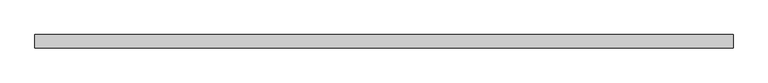
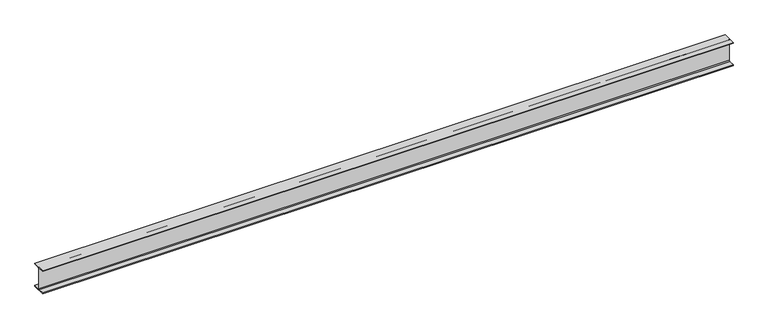
"""IFC4 building model written with IfcOpenShell, lengths in millimetres: beam geometry, Old_Steel Beam_H-KSD3502 : H_SB_ASB_H-300×300x10x15."""

from ifc_helpers import new_model, si_unit, point, frame, frame_2d, origin, place, context, project, spatial, polyline, circle_curve, trimmed, segment, composite_curve, outline, extrude, source, transform, mapped, element, save


def beam_81ff70bf(model_context):
    return source(origin(), model_context, "Body", "SweptSolid", [
        extrude(outline(composite_curve([segment(polyline([(-82.5, -141.5), (-11.9, -141.5)]), True, "CONTINUOUS"), segment(trimmed(circle_curve(frame_2d((-11.9, -132.6)), 8.9), [point((-11.9, -141.5))], [point((-3.0, -132.6))], True, "CARTESIAN"), True, "CONTINUOUS"), segment(polyline([(-3.0, -132.6), (-3.0, 132.6)]), True, "CONTINUOUS"), segment(trimmed(circle_curve(frame_2d((-11.9, 132.6)), 8.9), [point((-3.0, 132.6))], [point((-11.9, 141.5))], True, "CARTESIAN"), True, "CONTINUOUS"), segment(polyline([(-11.9, 141.5), (-82.5, 141.5), (-82.5, 151.7), (82.5, 151.7), (82.5, 141.5), (11.9, 141.5)]), True, "CONTINUOUS"), segment(trimmed(circle_curve(frame_2d((11.9, 132.6)), 8.9), [point((11.9, 141.5))], [point((3.0, 132.6))], True, "CARTESIAN"), True, "CONTINUOUS"), segment(polyline([(3.0, 132.6), (3.0, -132.6)]), True, "CONTINUOUS"), segment(trimmed(circle_curve(frame_2d((11.9, -132.6)), 8.9), [point((3.0, -132.6))], [point((11.9, -141.5))], True, "CARTESIAN"), True, "CONTINUOUS"), segment(polyline([(11.9, -141.5), (82.5, -141.5), (82.5, -151.7), (-82.5, -151.7), (-82.5, -141.5)]), True, "CONTINUOUS")], self_intersect=False)), frame((-4331.4958952, 0.0, 0.0), z_axis=(1.0, 0.0, 0.0), x_axis=(0.0, 1.0, 0.0)), (0.0, 0.0, 1.0), 8594.5528849),
    ])


if __name__ == "__main__":
    model = new_model("IFC4")
    model_context = context("Model", 3, world=origin())
    ifc_project = project(units=[si_unit("LENGTHUNIT", "METRE", prefix="MILLI")], contexts=[model_context])
    site = spatial("IfcSite", under=ifc_project)
    building = spatial("IfcBuilding", under=site)
    placement = place(None, origin())
    beam_shape = beam_81ff70bf(model_context)
    element("IfcBeam", 1, ObjectType="Old_Steel Beam_H-KSD3502 : H_SB_ASB_H-300×300x10x15", at=placement, inside=building, context=model_context, shape_type="MappedRepresentation", body=[
        mapped(beam_shape, transform((0.0, 0.0, 0.0), x_axis=(1.0, 0.0, 0.0), y_axis=(0.0, 1.0, 0.0), z_axis=(0.0, 0.0, 1.0))),
    ])
    save(model, "model.ifc")

# Revit data of these elements
# Type "Old_Steel Beam_H-KSD3502 : H_SB_ASB_H-300×300x10x15"
#   Width = 30.0 cm
#   Web Thickness = 1.0 cm
#   Web Fillet = 1.8 cm
#   Warping Constant = 1370670.0 cm⁶
#   Torsional Moment of Inertia = 77.00 cm⁴
#   Torsional Modulus = 1.0 cm³
#   Section Area = 119.8 cm²
#   Plastic Modulus weak axis = 684.0 cm³
#   Plastic Modulus strong axis = 1500.0 cm³
#   Perimeter = 1.75 m²/m
#   Nominal Weight = 94.00 kgf/m
#   Moment of Inertia weak axis = 6750.00 cm⁴
#   Moment of Inertia strong axis = 20400.00 cm⁴
#   Height = 30.0 cm
#   Flange Thickness = 1.5 cm
#   Elastic Modulus weak axis = 450.0 cm³
#   Elastic Modulus strong axis = 1360.0 cm³
#   Centroid Vertical = 15.0 cm
#   Centroid Horizontal = 15.0 cm
#   Length [instance default] = 1.5240 m
#   Structural Material [instance default] = Steel, 45-345
#   Assembly Code = ""
# Element 1 (IfcBeam, "Old_Steel Beam_H-KSD3502 : H_SB_ASB_H-300×300x10x15")
#   Structural Material = none
# Materials
#   "Steel, 45-345": class "Metal", colour RGB 189 187 185, transparency 0, Description = "Steel 345 MPa", Cost = 0
